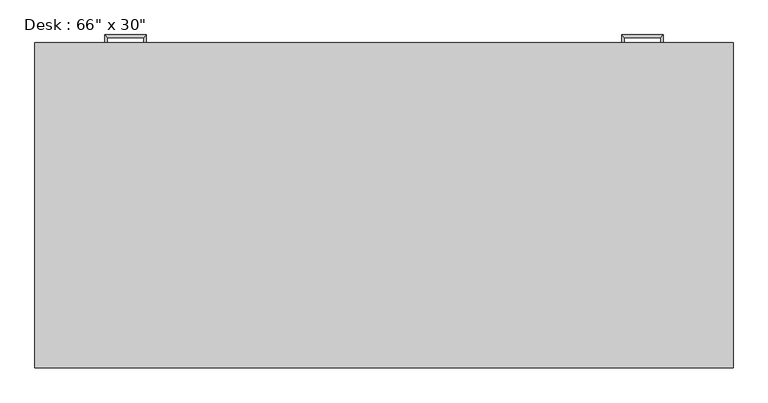
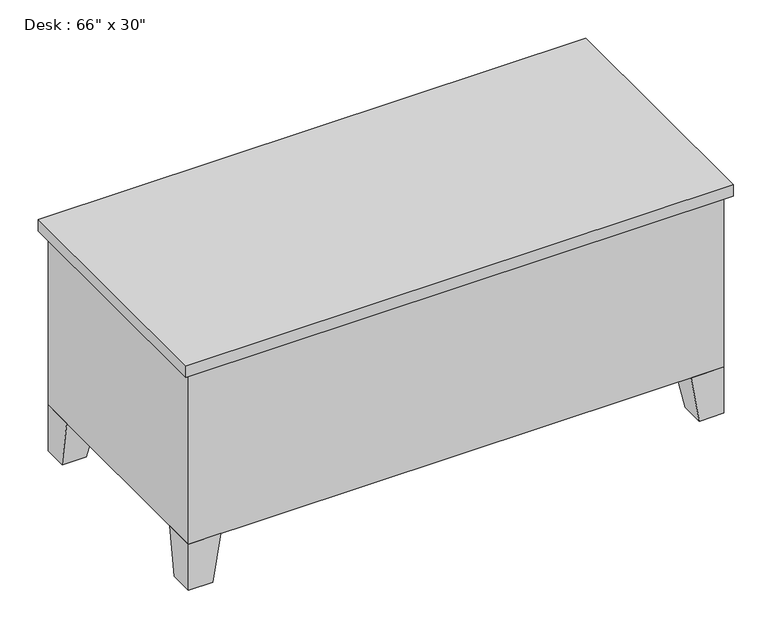
"""IFC4 building model written with IfcOpenShell, lengths in millimetres: furniture geometry."""

from ifc_helpers import new_model, si_unit, frame, origin, place, context, project, spatial, polyline, outline, extrude, faceted_brep, source, transform, mapped, element, save


def furniture_bcdaa455(model_context):
    return source(origin(), model_context, "Body", "SolidModel", [
        extrude(outline(polyline([(1657.35, 762.0), (1289.05, 762.0), (1289.05, 774.7), (1657.35, 774.7), (1657.35, 762.0)])), frame((0.0, 0.0, 603.25), z_axis=(0.0, 0.0, 1.0), x_axis=(1.0, 0.0, 0.0)), (0.0, 0.0, 1.0), 101.6),
        extrude(outline(polyline([(1657.35, 762.0), (1289.05, 762.0), (1289.05, 774.7), (1657.35, 774.7), (1657.35, 762.0)])), frame((0.0, 0.0, 171.45), z_axis=(0.0, 0.0, 1.0), x_axis=(1.0, 0.0, 0.0)), (0.0, 0.0, 1.0), 412.75),
        extrude(outline(polyline([(387.35, 762.0), (19.05, 762.0), (19.05, 774.7), (387.35, 774.7), (387.35, 762.0)])), frame((0.0, 0.0, 603.25), z_axis=(0.0, 0.0, 1.0), x_axis=(1.0, 0.0, 0.0)), (0.0, 0.0, 1.0), 101.6),
        extrude(outline(polyline([(387.35, 762.0), (19.05, 762.0), (19.05, 774.7), (387.35, 774.7), (387.35, 762.0)])), frame((0.0, 0.0, 171.45), z_axis=(0.0, 0.0, 1.0), x_axis=(1.0, 0.0, 0.0)), (0.0, 0.0, 1.0), 171.45),
        extrude(outline(polyline([(387.35, 762.0), (19.05, 762.0), (19.05, 774.7), (387.35, 774.7), (387.35, 762.0)])), frame((0.0, 0.0, 482.6), z_axis=(0.0, 0.0, 1.0), x_axis=(1.0, 0.0, 0.0)), (0.0, 0.0, 1.0), 101.6),
        extrude(outline(polyline([(387.35, 762.0), (19.05, 762.0), (19.05, 774.7), (387.35, 774.7), (387.35, 762.0)])), frame((0.0, 0.0, 361.95), z_axis=(0.0, 0.0, 1.0), x_axis=(1.0, 0.0, 0.0)), (0.0, 0.0, 1.0), 101.6),
        faceted_brep([(1574.8, 762.0, 152.4), (1574.8, 660.4, 152.4), (1676.4, 660.4, 152.4), (1676.4, 762.0, 152.4), (1600.2, 762.0, 0.0), (1676.4, 762.0, 0.0), (1676.4, 685.8, 0.0), (1600.2, 685.8, 0.0)], [[[0, 1, 2, 3]], [[4, 5, 6, 7]], [[4, 7, 1, 0]], [[7, 6, 2, 1]], [[6, 5, 3, 2]], [[5, 4, 0, 3]]]),
        faceted_brep([(1574.8, 0.0, 152.4), (1676.4, 0.0, 152.4), (1676.4, 101.6, 152.4), (1574.8, 101.6, 152.4), (1600.2, 0.0, 0.0), (1600.2, 76.2, 0.0), (1676.4, 76.2, 0.0), (1676.4, 0.0, 0.0)], [[[0, 1, 2, 3]], [[4, 5, 6, 7]], [[4, 7, 1, 0]], [[7, 6, 2, 1]], [[6, 5, 3, 2]], [[5, 4, 0, 3]]]),
        faceted_brep([(101.6, 0.0, 152.4), (101.6, 101.6, 152.4), (0.0, 101.6, 152.4), (0.0, 0.0, 152.4), (76.2, 0.0, 0.0), (0.0, 0.0, 0.0), (0.0, 76.2, 0.0), (76.2, 76.2, 0.0)], [[[0, 1, 2, 3]], [[4, 5, 6, 7]], [[4, 7, 1, 0]], [[7, 6, 2, 1]], [[6, 5, 3, 2]], [[5, 4, 0, 3]]]),
        faceted_brep([(101.6, 762.0, 152.4), (0.0, 762.0, 152.4), (0.0, 660.4, 152.4), (101.6, 660.4, 152.4), (76.2, 762.0, 0.0), (76.2, 685.8, 0.0), (0.0, 685.8, 0.0), (0.0, 762.0, 0.0)], [[[0, 1, 2, 3]], [[4, 5, 6, 7]], [[4, 7, 1, 0]], [[7, 6, 2, 1]], [[6, 5, 3, 2]], [[5, 4, 0, 3]]]),
        extrude(outline(polyline([(1695.45, 781.05), (1695.45, -19.05), (-19.05, -19.05), (-19.05, 781.05), (1695.45, 781.05)])), frame((0.0, 0.0, 723.9), z_axis=(0.0, 0.0, 1.0), x_axis=(1.0, 0.0, 0.0)), (0.0, 0.0, 1.0), 38.1),
        extrude(outline(polyline([(406.4, 762.0), (406.4, 50.8), (1270.0, 50.8), (1270.0, 762.0), (1676.4, 762.0), (1676.4, 0.0), (0.0, 0.0), (0.0, 762.0), (406.4, 762.0)])), frame((0.0, 0.0, 152.4), z_axis=(0.0, 0.0, 1.0), x_axis=(1.0, 0.0, 0.0)), (0.0, 0.0, 1.0), 571.5),
        faceted_brep([(1517.65, 774.7, 546.1), (1517.65, 774.7, 533.4), (1524.0, 774.7, 533.4), (1524.0, 774.7, 546.1), (1517.65, 793.75, 546.1), (1517.65, 793.75, 533.4), (1524.0, 800.1, 533.4), (1524.0, 800.1, 546.1), (1428.75, 793.75, 546.1), (1428.75, 793.75, 533.4), (1422.4, 800.1, 533.4), (1422.4, 800.1, 546.1), (1428.75, 774.7, 546.1), (1422.4, 774.7, 546.1), (1422.4, 774.7, 533.4), (1428.75, 774.7, 533.4)], [[[0, 1, 2, 3]], [[1, 0, 4, 5]], [[2, 1, 5, 6]], [[3, 2, 6, 7]], [[0, 3, 7, 4]], [[5, 4, 8, 9]], [[6, 5, 9, 10]], [[7, 6, 10, 11]], [[4, 7, 11, 8]], [[12, 13, 14, 15]], [[9, 8, 12, 15]], [[10, 9, 15, 14]], [[11, 10, 14, 13]], [[8, 11, 13, 12]]]),
        faceted_brep([(1517.65, 774.7, 666.75), (1517.65, 774.7, 654.05), (1524.0, 774.7, 654.05), (1524.0, 774.7, 666.75), (1517.65, 793.75, 666.75), (1517.65, 793.75, 654.05), (1524.0, 800.1, 654.05), (1524.0, 800.1, 666.75), (1428.75, 793.75, 666.75), (1428.75, 793.75, 654.05), (1422.4, 800.1, 654.05), (1422.4, 800.1, 666.75), (1428.75, 774.7, 666.75), (1422.4, 774.7, 666.75), (1422.4, 774.7, 654.05), (1428.75, 774.7, 654.05)], [[[0, 1, 2, 3]], [[1, 0, 4, 5]], [[2, 1, 5, 6]], [[3, 2, 6, 7]], [[0, 3, 7, 4]], [[5, 4, 8, 9]], [[6, 5, 9, 10]], [[7, 6, 10, 11]], [[4, 7, 11, 8]], [[12, 13, 14, 15]], [[9, 8, 12, 15]], [[10, 9, 15, 14]], [[11, 10, 14, 13]], [[8, 11, 13, 12]]]),
        faceted_brep([(158.75, 774.7, 304.8), (152.4, 774.7, 304.8), (152.4, 774.7, 292.1), (158.75, 774.7, 292.1), (158.75, 793.75, 304.8), (152.4, 800.1, 304.8), (152.4, 800.1, 292.1), (158.75, 793.75, 292.1), (247.65, 793.75, 304.8), (254.0, 800.1, 304.8), (254.0, 800.1, 292.1), (247.65, 793.75, 292.1), (247.65, 774.7, 304.8), (247.65, 774.7, 292.1), (254.0, 774.7, 292.1), (254.0, 774.7, 304.8)], [[[0, 1, 2, 3]], [[1, 0, 4, 5]], [[2, 1, 5, 6]], [[3, 2, 6, 7]], [[0, 3, 7, 4]], [[5, 4, 8, 9]], [[6, 5, 9, 10]], [[7, 6, 10, 11]], [[4, 7, 11, 8]], [[12, 13, 14, 15]], [[9, 8, 12, 15]], [[10, 9, 15, 14]], [[11, 10, 14, 13]], [[8, 11, 13, 12]]]),
        faceted_brep([(158.75, 774.7, 425.45), (152.4, 774.7, 425.45), (152.4, 774.7, 412.75), (158.75, 774.7, 412.75), (158.75, 793.75, 425.45), (152.4, 800.1, 425.45), (152.4, 800.1, 412.75), (158.75, 793.75, 412.75), (247.65, 793.75, 425.45), (254.0, 800.1, 425.45), (254.0, 800.1, 412.75), (247.65, 793.75, 412.75), (247.65, 774.7, 425.45), (247.65, 774.7, 412.75), (254.0, 774.7, 412.75), (254.0, 774.7, 425.45)], [[[0, 1, 2, 3]], [[1, 0, 4, 5]], [[2, 1, 5, 6]], [[3, 2, 6, 7]], [[0, 3, 7, 4]], [[5, 4, 8, 9]], [[6, 5, 9, 10]], [[7, 6, 10, 11]], [[4, 7, 11, 8]], [[12, 13, 14, 15]], [[9, 8, 12, 15]], [[10, 9, 15, 14]], [[11, 10, 14, 13]], [[8, 11, 13, 12]]]),
        faceted_brep([(158.75, 774.7, 546.1), (152.4, 774.7, 546.1), (152.4, 774.7, 533.4), (158.75, 774.7, 533.4), (158.75, 793.75, 546.1), (152.4, 800.1, 546.1), (152.4, 800.1, 533.4), (158.75, 793.75, 533.4), (247.65, 793.75, 546.1), (254.0, 800.1, 546.1), (254.0, 800.1, 533.4), (247.65, 793.75, 533.4), (247.65, 774.7, 546.1), (247.65, 774.7, 533.4), (254.0, 774.7, 533.4), (254.0, 774.7, 546.1)], [[[0, 1, 2, 3]], [[1, 0, 4, 5]], [[2, 1, 5, 6]], [[3, 2, 6, 7]], [[0, 3, 7, 4]], [[5, 4, 8, 9]], [[6, 5, 9, 10]], [[7, 6, 10, 11]], [[4, 7, 11, 8]], [[12, 13, 14, 15]], [[9, 8, 12, 15]], [[10, 9, 15, 14]], [[11, 10, 14, 13]], [[8, 11, 13, 12]]]),
        faceted_brep([(158.75, 774.7, 666.75), (152.4, 774.7, 666.75), (152.4, 774.7, 654.05), (158.75, 774.7, 654.05), (158.75, 793.75, 666.75), (152.4, 800.1, 666.75), (152.4, 800.1, 654.05), (158.75, 793.75, 654.05), (247.65, 793.75, 666.75), (254.0, 800.1, 666.75), (254.0, 800.1, 654.05), (247.65, 793.75, 654.05), (247.65, 774.7, 666.75), (247.65, 774.7, 654.05), (254.0, 774.7, 654.05), (254.0, 774.7, 666.75)], [[[0, 1, 2, 3]], [[1, 0, 4, 5]], [[2, 1, 5, 6]], [[3, 2, 6, 7]], [[0, 3, 7, 4]], [[5, 4, 8, 9]], [[6, 5, 9, 10]], [[7, 6, 10, 11]], [[4, 7, 11, 8]], [[12, 13, 14, 15]], [[9, 8, 12, 15]], [[10, 9, 15, 14]], [[11, 10, 14, 13]], [[8, 11, 13, 12]]]),
    ])


if __name__ == "__main__":
    model = new_model("IFC4")
    model_context = context("Model", 3, world=origin())
    ifc_project = project(units=[si_unit("LENGTHUNIT", "METRE", prefix="MILLI")], contexts=[model_context])
    site = spatial("IfcSite", under=ifc_project)
    building = spatial("IfcBuilding", under=site)
    placement = place(None, origin())
    furniture_shape = furniture_bcdaa455(model_context)
    element("IfcFurniture", 1, ObjectType="Desk : 66\" x 30\"", at=placement, inside=building, context=model_context, shape_type="MappedRepresentation", body=[
        mapped(furniture_shape, transform((0.0, 0.0, 0.0), x_axis=(1.0, 0.0, 0.0), y_axis=(0.0, 1.0, 0.0), z_axis=(0.0, 0.0, 1.0))),
    ])
    save(model, "model.ifc")

# Revit data of these elements
# Type "Desk : 66\" x 30\""
#   Model = "TSK-5679"
#   Manufacturer = "Acme Furniture"
#   Type Mark = "DK-2"
#   Assembly Code = "E2020200"
#   Cost = 1050
#   Depth = 2' - 6"
#   Height = 2' - 6"
#   Leg Height = 0' - 6"
#   Width = 5' - 6"
#   Body Material = Laminate, Ivory, Matte
#   Handle/Leg Material = Steel, Chrome Plated
#   Top Material = Cherry
#   Default Elevation = 0
# Element 1 (IfcFurniture, "Desk : 66\" x 30\"")
#   Materials on its faces: "Steel, Chrome Plated", "Laminate, Ivory, Matte", "Cherry"
# Materials
#   "Laminate, Ivory, Matte": class "Plastic", colour RGB 247 247 239, transparency 0, Description = "Plastic Laminate - Ivory, Matte", Cost = 0
#   "Steel, Chrome Plated": class "Metal", colour RGB 17 17 17, transparency 0, Description = "Chromiuim plated steel", Cost = 0
#   "Cherry": class "Wood", colour RGB 226 177 128, transparency 0, Description = "Prunus Serotina", Cost = 0
